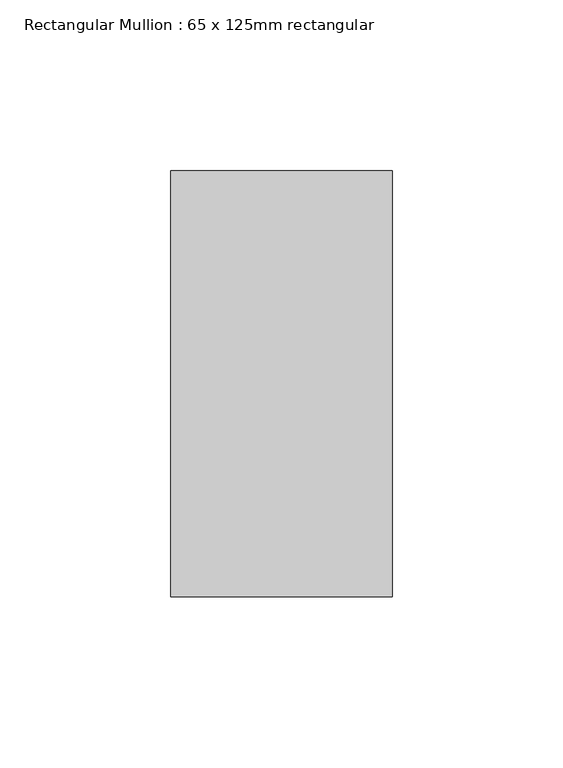
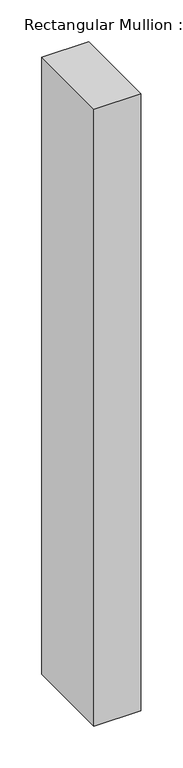
"""IFC4 building model written with IfcOpenShell, lengths in millimetres: member geometry, Rectangular Mullion : 65 x 125mm rectangular."""

from ifc_helpers import new_model, si_unit, frame, origin, place, context, project, spatial, polyline, outline, extrude, source, transform, mapped, element, save


def rectangular_mullion_65_x_125mm_rectangular_9a77bebc(model_context):
    return source(origin(), model_context, "Body", "SweptSolid", [
        extrude(outline(polyline([(0.0, 62.5), (0.0, -62.5), (-65.0, -62.5), (-65.0, 62.5), (0.0, 62.5)])), frame((0.0, 0.0, -902.5000003), z_axis=(0.0, 0.0, 1.0), x_axis=(1.0, 0.0, 0.0)), (0.0, 0.0, 1.0), 902.5000003),
    ])


if __name__ == "__main__":
    model = new_model("IFC4")
    model_context = context("Model", 3, world=origin())
    ifc_project = project(units=[si_unit("LENGTHUNIT", "METRE", prefix="MILLI")], contexts=[model_context])
    site = spatial("IfcSite", under=ifc_project)
    building = spatial("IfcBuilding", under=site)
    placement = place(None, origin())
    rectangular_mullion_65_x_125mm_rectangular_shape = rectangular_mullion_65_x_125mm_rectangular_9a77bebc(model_context)
    element("IfcMember", 1, ObjectType="Rectangular Mullion : 65 x 125mm rectangular", at=placement, inside=building, context=model_context, shape_type="MappedRepresentation", body=[
        mapped(rectangular_mullion_65_x_125mm_rectangular_shape, transform((0.0, 0.0, 0.0), x_axis=(1.0, 0.0, 0.0), y_axis=(0.0, 1.0, 0.0), z_axis=(0.0, 0.0, 1.0))),
    ])
    save(model, "model.ifc")

# Revit data of these elements
# Type "Rectangular Mullion : 65 x 125mm rectangular"
#   built-in parameter 1007304 = 0.410105 (stored number, unit not read)
#   built-in parameter 1007301 = 0.106627 (stored number, unit not read)
#   built-in parameter 1007300 = 0.106627 (stored number, unit not read)
# Element 1 (IfcMember, "Rectangular Mullion : 65 x 125mm rectangular")
#   Materials on its faces: "Aluminum"
# Materials
#   "Aluminum": class "Metal", colour RGB 244 245 246, transparency 0, Description = "Aluminum 6061", Cost = 0
